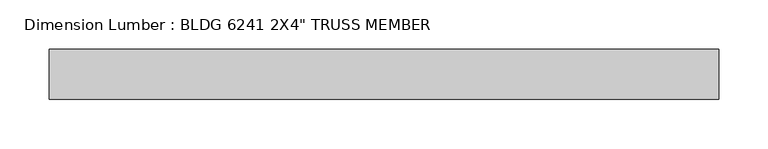
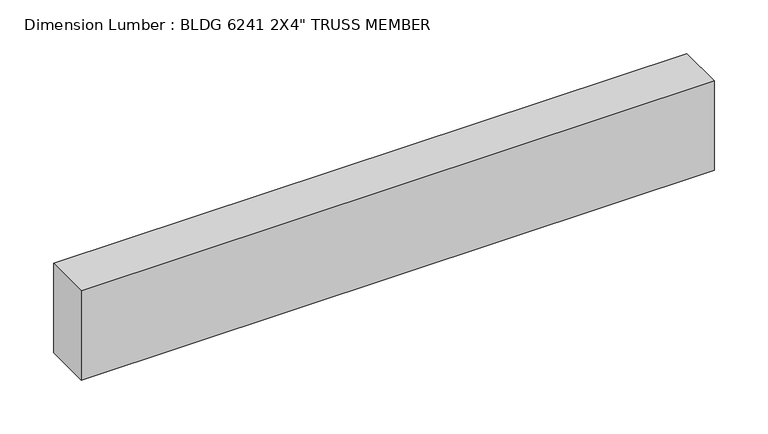
"""IFC4 building model written with IfcOpenShell, lengths in millimetres: beam geometry."""

import ifcopenshell
import ifcopenshell.guid

model = None  # the IFC model being written
_history = None  # IfcOwnerHistory: only IFC2X3 demands one
_inside = {}  # id of a spatial element -> (the spatial element, [elements in it])
_under = {}  # id of a project, library or spatial element -> (it, [spatial elements below it])
_declared = {}  # id of a project -> (the project, [libraries it declares])
_typed = {}  # id of a type object -> (the type object, [elements of that type])
_made_of = {}  # id of a material, layer set ... -> (it, [elements and type objects made of it])


def new_model(schema):
    """Start an empty IFC model of exactly this schema.

    Asked for "IFC4X3", IfcOpenShell would pick the latest addendum, in which some entities
    have other attributes; the version numbers below select the first issue.
    IFC2X3 requires an IfcOwnerHistory on every rooted entity: one is made here for all.
    """
    global model, _history
    if schema == "IFC4X3":
        model = ifcopenshell.file(schema_version=(4, 3, 0, 0))
    else:
        model = ifcopenshell.file(schema=schema)
    _inside.clear()
    _under.clear()
    _declared.clear()
    _typed.clear()
    _made_of.clear()
    _history = None
    if model.schema == "IFC2X3":
        org = make("IfcOrganization", Name="unknown")
        user = make(
            "IfcPersonAndOrganization",
            ThePerson=make("IfcPerson", FamilyName="unknown"),
            TheOrganization=org,
        )
        app = make(
            "IfcApplication",
            ApplicationDeveloper=org,
            Version="unknown",
            ApplicationFullName="unknown",
            ApplicationIdentifier="unknown",
        )
        _history = make(
            "IfcOwnerHistory",
            OwningUser=user,
            OwningApplication=app,
            ChangeAction="ADDED",
            CreationDate=0,
        )
    return model


def make(cls, **values):
    """One entity of the class cls with the attributes given. An attribute that is None is left unset."""
    return model.create_entity(
        cls, **{name: value for name, value in values.items() if value is not None}
    )


def rooted(cls, **values):
    """An entity with a GlobalId (a new one), such as an element, a storey or a relation."""
    return make(cls, GlobalId=ifcopenshell.guid.new(), OwnerHistory=_history, **values)


def si_unit(unit_type, name, prefix=None):
    """IfcSIUnit, for example si_unit("LENGTHUNIT", "METRE", prefix="MILLI")."""
    return make("IfcSIUnit", UnitType=unit_type, Prefix=prefix, Name=name)


def assignment(units):
    """IfcUnitAssignment: the units of a project."""
    return None if units is None else make("IfcUnitAssignment", Units=units)


def point(xyz):
    """IfcCartesianPoint."""
    return None if xyz is None else make("IfcCartesianPoint", Coordinates=xyz)


def direction(xyz):
    """IfcDirection."""
    return None if xyz is None else make("IfcDirection", DirectionRatios=xyz)


def frame(location, z_axis=None, x_axis=None):
    """IfcAxis2Placement3D, a coordinate frame: its origin and axes. An axis left out is left unset."""
    return make(
        "IfcAxis2Placement3D",
        Location=point(location),
        Axis=direction(z_axis),
        RefDirection=direction(x_axis),
    )


def origin():
    """The frame at (0, 0, 0) with its axes left unset."""
    return frame((0.0, 0.0, 0.0))


def place(relative_to, where):
    """IfcLocalPlacement: puts the frame where relative to a parent placement (None: the world)."""
    return make(
        "IfcLocalPlacement", PlacementRelTo=relative_to, RelativePlacement=where
    )


def context(
    kind, dimensions, precision=None, world=None, true_north=None, identifier=None
):
    """IfcGeometricRepresentationContext, for example the 3D "Model" context."""
    return make(
        "IfcGeometricRepresentationContext",
        ContextIdentifier=identifier,
        ContextType=kind,
        CoordinateSpaceDimension=dimensions,
        Precision=precision,
        WorldCoordinateSystem=world,
        TrueNorth=true_north,
    )


def project(units=None, contexts=None):
    """IfcProject with its units and contexts."""
    return rooted(
        "IfcProject",
        Name="project",
        RepresentationContexts=contexts,
        UnitsInContext=assignment(units),
    )


def spatial(cls, under=None, at=None, **own):
    """A site, building, storey or space (cls), placed at a placement, below another one or the project."""
    s = rooted(cls, ObjectPlacement=at, **own)
    if under is not None:
        _under.setdefault(under.id(), (under, []))[1].append(s)
    return s


def polyline(points):
    """IfcPolyline through the points."""
    return make("IfcPolyline", Points=[point(p) for p in points])


def outline(outer, holes=None, kind="AREA"):
    """IfcArbitraryClosedProfileDef: a profile drawn as a closed curve; with holes, ...WithVoids."""
    if holes is None:
        return make("IfcArbitraryClosedProfileDef", ProfileType=kind, OuterCurve=outer)
    return make(
        "IfcArbitraryProfileDefWithVoids",
        ProfileType=kind,
        OuterCurve=outer,
        InnerCurves=holes,
    )


def extrude(swept, where, along, depth):
    """IfcExtrudedAreaSolid: the profile swept, set in the frame where, extruded along a direction by depth."""
    return make(
        "IfcExtrudedAreaSolid",
        SweptArea=swept,
        Position=where,
        ExtrudedDirection=direction(along),
        Depth=depth,
    )


def shape(context_of_items, identifier, shape_type, items):
    """IfcShapeRepresentation: the items that make up one representation, for example the "Body"."""
    return make(
        "IfcShapeRepresentation",
        ContextOfItems=context_of_items,
        RepresentationIdentifier=identifier,
        RepresentationType=shape_type,
        Items=items,
    )


def source(mapping_origin, context_of_items, identifier, shape_type, items):
    """IfcRepresentationMap: a shape defined once, which mapped items show again and again."""
    return make(
        "IfcRepresentationMap",
        MappingOrigin=mapping_origin,
        MappedRepresentation=shape(context_of_items, identifier, shape_type, items),
    )


def transform(
    local_origin,
    x_axis=None,
    y_axis=None,
    z_axis=None,
    scale=None,
    scale2=None,
    scale3=None,
    uniform=True,
):
    """IfcCartesianTransformationOperator3D, or its non-uniform kind. x_axis, y_axis, z_axis: its Axis1, 2, 3."""
    if uniform:
        return make(
            "IfcCartesianTransformationOperator3D",
            Axis1=direction(x_axis),
            Axis2=direction(y_axis),
            LocalOrigin=point(local_origin),
            Scale=scale,
            Axis3=direction(z_axis),
        )
    return make(
        "IfcCartesianTransformationOperator3DnonUniform",
        Axis1=direction(x_axis),
        Axis2=direction(y_axis),
        LocalOrigin=point(local_origin),
        Scale=scale,
        Axis3=direction(z_axis),
        Scale2=scale2,
        Scale3=scale3,
    )


def mapped(mapping_source, mapping_target):
    """IfcMappedItem: shows the shape of a source again, moved by a transform."""
    return make(
        "IfcMappedItem", MappingSource=mapping_source, MappingTarget=mapping_target
    )


def made_of(thing, what):
    """Note that an element or type object is made of a material, layer set ...; save() writes the relation."""
    if what is not None:
        _made_of.setdefault(what.id(), (what, []))[1].append(thing)
    return thing


def element(
    cls,
    number,
    at=None,
    inside=None,
    cuts=None,
    type_object=None,
    material=None,
    context=None,
    identifier="Body",
    shape_type=None,
    held_by="IfcProductDefinitionShape",
    body=None,
    shapes=None,
    **own,
):
    """One element of the class cls, such as IfcWall. Its Tag is "e" and its number.

    at: its placement. inside: the storey or other place that contains it. cuts: it is an
    opening in that element (IfcRelVoidsElement). A single representation is given by context,
    identifier, shape_type and body (its items); several are given by shapes. held_by: the class
    of the entity that holds the representations. save() writes the other relations.
    """
    e = rooted(cls, Tag="e%d" % number, ObjectPlacement=at, **own)
    if body is not None:
        shapes = [shape(context, identifier, shape_type, body)]
    if shapes is not None:
        e.Representation = make(held_by, Representations=shapes)
    if inside is not None:
        _inside.setdefault(inside.id(), (inside, []))[1].append(e)
    if cuts is not None:
        rooted(
            "IfcRelVoidsElement", RelatingBuildingElement=cuts, RelatedOpeningElement=e
        )
    if type_object is not None:
        _typed.setdefault(type_object.id(), (type_object, []))[1].append(e)
    return made_of(e, material)


def aggregate(whole, parts):
    """IfcRelAggregates: a whole, such as a stair, and the parts it consists of."""
    return rooted("IfcRelAggregates", RelatingObject=whole, RelatedObjects=parts)


def save(model, path):
    """Write the relations noted so far, then the file.

    IfcRelAggregates (storeys below a building ...), IfcRelContainedInSpatialStructure (elements
    in a storey), IfcRelDefinesByType, IfcRelAssociatesMaterial and IfcRelDeclares: one each for
    every whole, place, type object, material and project.
    """
    for whole, parts in _under.values():
        aggregate(whole, parts)
    for where, things in _inside.values():
        rooted(
            "IfcRelContainedInSpatialStructure",
            RelatedElements=things,
            RelatingStructure=where,
        )
    for kind, things in _typed.values():
        rooted("IfcRelDefinesByType", RelatedObjects=things, RelatingType=kind)
    for what, things in _made_of.values():
        rooted("IfcRelAssociatesMaterial", RelatedObjects=things, RelatingMaterial=what)
    for by, libraries in _declared.values():
        rooted("IfcRelDeclares", RelatingContext=by, RelatedDefinitions=libraries)
    model.write(path)


def beam_78ff79ac(model_context):
    return source(origin(), model_context, "Body", "SweptSolid", [
        extrude(outline(polyline([(365.3019367, -25.4), (-314.5019367, -25.4), (-314.5019367, 25.4), (365.3019367, 25.4), (365.3019367, -25.4)])), frame((0.0, 0.0, -50.8), z_axis=(0.0, 0.0, 1.0), x_axis=(1.0, 0.0, 0.0)), (0.0, 0.0, 1.0), 101.6),
    ])


if __name__ == "__main__":
    model = new_model("IFC4")
    model_context = context("Model", 3, world=origin())
    ifc_project = project(units=[si_unit("LENGTHUNIT", "METRE", prefix="MILLI")], contexts=[model_context])
    site = spatial("IfcSite", under=ifc_project)
    building = spatial("IfcBuilding", under=site)
    placement = place(None, origin())
    beam_shape = beam_78ff79ac(model_context)
    element("IfcBeam", 1, ObjectType="Dimension Lumber : BLDG 6241 2X4\" TRUSS MEMBER", at=placement, inside=building, context=model_context, shape_type="MappedRepresentation", body=[
        mapped(beam_shape, transform((0.0, 0.0, 0.0), x_axis=(1.0, 0.0, 0.0), y_axis=(0.0, 1.0, 0.0), z_axis=(0.0, 0.0, 1.0))),
    ])
    save(model, "model.ifc")

# Revit data of these elements
# Type "Dimension Lumber : BLDG 6241 2X4\" TRUSS MEMBER"
#   Assembly Code = "B10"
#   A = 0.273472 SF
#   Length [instance default] = 5' - 0"
#   b = 0' - 2"
#   d = 0' - 4"
#   Structural Material [instance default] = Softwood, Lumber
# Element 1 (IfcBeam, "Dimension Lumber : BLDG 6241 2X4\" TRUSS MEMBER")
#   Materials on its faces: "Softwood, Lumber"
# Materials
#   "Softwood, Lumber": class "Wood", colour RGB 223 192 134, transparency 0, Description = "Pinus Echinata", Cost = 0
